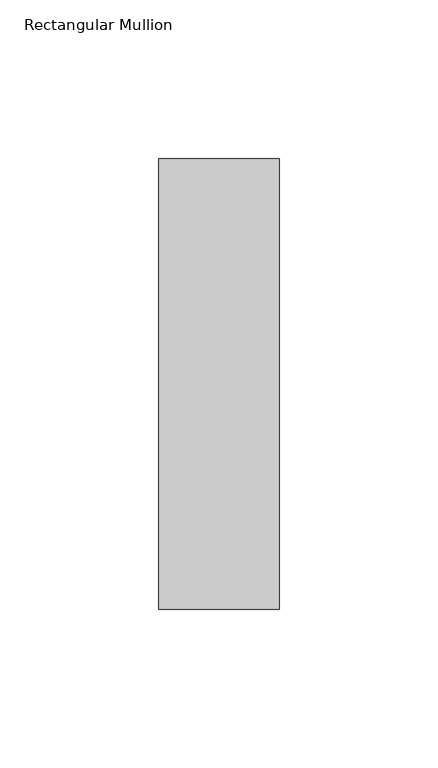
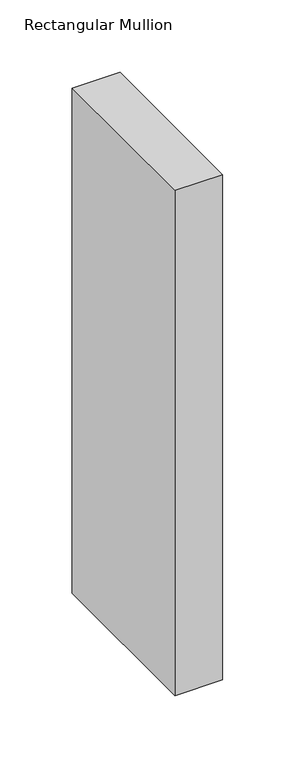
"""IFC4 building model written with IfcOpenShell, lengths in millimetres: member geometry, Rectangular Mullion : NLRS_21_CWM_hsb-regel 38x142_gen_rsf."""

from ifc_helpers import new_model, si_unit, frame, origin, place, context, project, spatial, polyline, outline, extrude, source, transform, mapped, element, save


def rectangular_mullion_4d4fc8f4(model_context):
    return source(origin(), model_context, "Body", "SweptSolid", [
        extrude(outline(polyline([(0.0, -71.0), (-38.0, -71.0), (-38.0, 71.0), (0.0, 71.0), (0.0, -71.0)])), frame((0.0, 0.0, -426.0), z_axis=(0.0, 0.0, 1.0), x_axis=(1.0, 0.0, 0.0)), (0.0, 0.0, 1.0), 426.0),
    ])


if __name__ == "__main__":
    model = new_model("IFC4")
    model_context = context("Model", 3, world=origin())
    ifc_project = project(units=[si_unit("LENGTHUNIT", "METRE", prefix="MILLI")], contexts=[model_context])
    site = spatial("IfcSite", under=ifc_project)
    building = spatial("IfcBuilding", under=site)
    placement = place(None, origin())
    rectangular_mullion_shape = rectangular_mullion_4d4fc8f4(model_context)
    element("IfcMember", 1, ObjectType="Rectangular Mullion : NLRS_21_CWM_hsb-regel 38x142_gen_rsf", at=placement, inside=building, context=model_context, shape_type="MappedRepresentation", body=[
        mapped(rectangular_mullion_shape, transform((0.0, 0.0, 0.0), x_axis=(1.0, 0.0, 0.0), y_axis=(0.0, 1.0, 0.0), z_axis=(0.0, 0.0, 1.0))),
    ])
    save(model, "model.ifc")

# Revit data of these elements
# Type "Rectangular Mullion : NLRS_21_CWM_hsb-regel 38x142_gen_rsf"
#   Export Type to IFC As = "IfcWall"
#   Type IfcGUID = "07M7mRoiH1CR8m_RSKIwpF"
#   Assembly Code = "21.10"
#   built-in parameter 1007322 = 0.465879 (stored number, unit not read)
#   built-in parameter 1007321 = 0.062336 (stored number, unit not read)
#   built-in parameter 1007320 = 0.062336 (stored number, unit not read)
# Element 1 (IfcMember, "Rectangular Mullion : NLRS_21_CWM_hsb-regel 38x142_gen_rsf")
#   Materials on its faces: "NLRS_i2_hout naaldhout vuren_gen_rsf"
# Materials
#   "NLRS_i2_hout naaldhout vuren_gen_rsf": class "I - Hout", colour RGB 234 199 147, transparency 0, Keynote = "i2", Manufacturer = "Revit Standards Foundation", URL = "www.revitstandards.org", Description = "hout vuren", Cost = 0
